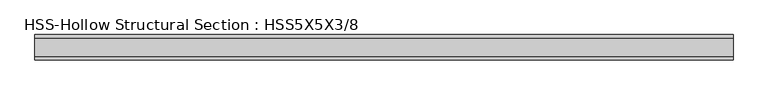
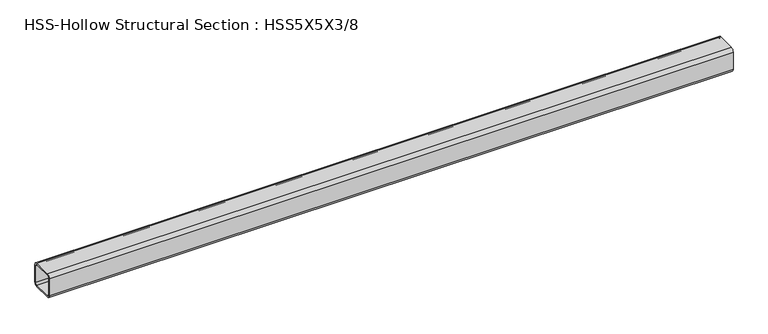
"""IFC4 building model written with IfcOpenShell, lengths in millimetres: member geometry, HSS-Hollow Structural Section : HSS5X5X3/8."""

import ifcopenshell
import ifcopenshell.guid

model = None  # the IFC model being written
_history = None  # IfcOwnerHistory: only IFC2X3 demands one
_inside = {}  # id of a spatial element -> (the spatial element, [elements in it])
_under = {}  # id of a project, library or spatial element -> (it, [spatial elements below it])
_declared = {}  # id of a project -> (the project, [libraries it declares])
_typed = {}  # id of a type object -> (the type object, [elements of that type])
_made_of = {}  # id of a material, layer set ... -> (it, [elements and type objects made of it])


def new_model(schema):
    """Start an empty IFC model of exactly this schema.

    Asked for "IFC4X3", IfcOpenShell would pick the latest addendum, in which some entities
    have other attributes; the version numbers below select the first issue.
    IFC2X3 requires an IfcOwnerHistory on every rooted entity: one is made here for all.
    """
    global model, _history
    if schema == "IFC4X3":
        model = ifcopenshell.file(schema_version=(4, 3, 0, 0))
    else:
        model = ifcopenshell.file(schema=schema)
    _inside.clear()
    _under.clear()
    _declared.clear()
    _typed.clear()
    _made_of.clear()
    _history = None
    if model.schema == "IFC2X3":
        org = make("IfcOrganization", Name="unknown")
        user = make(
            "IfcPersonAndOrganization",
            ThePerson=make("IfcPerson", FamilyName="unknown"),
            TheOrganization=org,
        )
        app = make(
            "IfcApplication",
            ApplicationDeveloper=org,
            Version="unknown",
            ApplicationFullName="unknown",
            ApplicationIdentifier="unknown",
        )
        _history = make(
            "IfcOwnerHistory",
            OwningUser=user,
            OwningApplication=app,
            ChangeAction="ADDED",
            CreationDate=0,
        )
    return model


def make(cls, **values):
    """One entity of the class cls with the attributes given. An attribute that is None is left unset."""
    return model.create_entity(
        cls, **{name: value for name, value in values.items() if value is not None}
    )


def rooted(cls, **values):
    """An entity with a GlobalId (a new one), such as an element, a storey or a relation."""
    return make(cls, GlobalId=ifcopenshell.guid.new(), OwnerHistory=_history, **values)


def si_unit(unit_type, name, prefix=None):
    """IfcSIUnit, for example si_unit("LENGTHUNIT", "METRE", prefix="MILLI")."""
    return make("IfcSIUnit", UnitType=unit_type, Prefix=prefix, Name=name)


def assignment(units):
    """IfcUnitAssignment: the units of a project."""
    return None if units is None else make("IfcUnitAssignment", Units=units)


def point(xyz):
    """IfcCartesianPoint."""
    return None if xyz is None else make("IfcCartesianPoint", Coordinates=xyz)


def direction(xyz):
    """IfcDirection."""
    return None if xyz is None else make("IfcDirection", DirectionRatios=xyz)


def frame(location, z_axis=None, x_axis=None):
    """IfcAxis2Placement3D, a coordinate frame: its origin and axes. An axis left out is left unset."""
    return make(
        "IfcAxis2Placement3D",
        Location=point(location),
        Axis=direction(z_axis),
        RefDirection=direction(x_axis),
    )


def frame_2d(location, x_axis=None):
    """IfcAxis2Placement2D, a coordinate frame in the plane: its origin and x axis."""
    return make(
        "IfcAxis2Placement2D", Location=point(location), RefDirection=direction(x_axis)
    )


def origin():
    """The frame at (0, 0, 0) with its axes left unset."""
    return frame((0.0, 0.0, 0.0))


def place(relative_to, where):
    """IfcLocalPlacement: puts the frame where relative to a parent placement (None: the world)."""
    return make(
        "IfcLocalPlacement", PlacementRelTo=relative_to, RelativePlacement=where
    )


def context(
    kind, dimensions, precision=None, world=None, true_north=None, identifier=None
):
    """IfcGeometricRepresentationContext, for example the 3D "Model" context."""
    return make(
        "IfcGeometricRepresentationContext",
        ContextIdentifier=identifier,
        ContextType=kind,
        CoordinateSpaceDimension=dimensions,
        Precision=precision,
        WorldCoordinateSystem=world,
        TrueNorth=true_north,
    )


def project(units=None, contexts=None):
    """IfcProject with its units and contexts."""
    return rooted(
        "IfcProject",
        Name="project",
        RepresentationContexts=contexts,
        UnitsInContext=assignment(units),
    )


def spatial(cls, under=None, at=None, **own):
    """A site, building, storey or space (cls), placed at a placement, below another one or the project."""
    s = rooted(cls, ObjectPlacement=at, **own)
    if under is not None:
        _under.setdefault(under.id(), (under, []))[1].append(s)
    return s


def polyline(points):
    """IfcPolyline through the points."""
    return make("IfcPolyline", Points=[point(p) for p in points])


def circle_curve(where, radius):
    """IfcCircle in the frame where."""
    return make("IfcCircle", Position=where, Radius=radius)


def trimmed(basis, trim1, trim2, sense, master):
    """IfcTrimmedCurve: the piece of a basis curve between two trims."""
    return make(
        "IfcTrimmedCurve",
        BasisCurve=basis,
        Trim1=trim1,
        Trim2=trim2,
        SenseAgreement=sense,
        MasterRepresentation=master,
    )


def segment(curve, same_sense, transition):
    """IfcCompositeCurveSegment."""
    return make(
        "IfcCompositeCurveSegment",
        Transition=transition,
        SameSense=same_sense,
        ParentCurve=curve,
    )


def composite_curve(segments, self_intersect=None):
    """IfcCompositeCurve: segments joined end to end."""
    return make("IfcCompositeCurve", Segments=segments, SelfIntersect=self_intersect)


def outline(outer, holes=None, kind="AREA"):
    """IfcArbitraryClosedProfileDef: a profile drawn as a closed curve; with holes, ...WithVoids."""
    if holes is None:
        return make("IfcArbitraryClosedProfileDef", ProfileType=kind, OuterCurve=outer)
    return make(
        "IfcArbitraryProfileDefWithVoids",
        ProfileType=kind,
        OuterCurve=outer,
        InnerCurves=holes,
    )


def extrude(swept, where, along, depth):
    """IfcExtrudedAreaSolid: the profile swept, set in the frame where, extruded along a direction by depth."""
    return make(
        "IfcExtrudedAreaSolid",
        SweptArea=swept,
        Position=where,
        ExtrudedDirection=direction(along),
        Depth=depth,
    )


def shape(context_of_items, identifier, shape_type, items):
    """IfcShapeRepresentation: the items that make up one representation, for example the "Body"."""
    return make(
        "IfcShapeRepresentation",
        ContextOfItems=context_of_items,
        RepresentationIdentifier=identifier,
        RepresentationType=shape_type,
        Items=items,
    )


def source(mapping_origin, context_of_items, identifier, shape_type, items):
    """IfcRepresentationMap: a shape defined once, which mapped items show again and again."""
    return make(
        "IfcRepresentationMap",
        MappingOrigin=mapping_origin,
        MappedRepresentation=shape(context_of_items, identifier, shape_type, items),
    )


def transform(
    local_origin,
    x_axis=None,
    y_axis=None,
    z_axis=None,
    scale=None,
    scale2=None,
    scale3=None,
    uniform=True,
):
    """IfcCartesianTransformationOperator3D, or its non-uniform kind. x_axis, y_axis, z_axis: its Axis1, 2, 3."""
    if uniform:
        return make(
            "IfcCartesianTransformationOperator3D",
            Axis1=direction(x_axis),
            Axis2=direction(y_axis),
            LocalOrigin=point(local_origin),
            Scale=scale,
            Axis3=direction(z_axis),
        )
    return make(
        "IfcCartesianTransformationOperator3DnonUniform",
        Axis1=direction(x_axis),
        Axis2=direction(y_axis),
        LocalOrigin=point(local_origin),
        Scale=scale,
        Axis3=direction(z_axis),
        Scale2=scale2,
        Scale3=scale3,
    )


def mapped(mapping_source, mapping_target):
    """IfcMappedItem: shows the shape of a source again, moved by a transform."""
    return make(
        "IfcMappedItem", MappingSource=mapping_source, MappingTarget=mapping_target
    )


def made_of(thing, what):
    """Note that an element or type object is made of a material, layer set ...; save() writes the relation."""
    if what is not None:
        _made_of.setdefault(what.id(), (what, []))[1].append(thing)
    return thing


def element(
    cls,
    number,
    at=None,
    inside=None,
    cuts=None,
    type_object=None,
    material=None,
    context=None,
    identifier="Body",
    shape_type=None,
    held_by="IfcProductDefinitionShape",
    body=None,
    shapes=None,
    **own,
):
    """One element of the class cls, such as IfcWall. Its Tag is "e" and its number.

    at: its placement. inside: the storey or other place that contains it. cuts: it is an
    opening in that element (IfcRelVoidsElement). A single representation is given by context,
    identifier, shape_type and body (its items); several are given by shapes. held_by: the class
    of the entity that holds the representations. save() writes the other relations.
    """
    e = rooted(cls, Tag="e%d" % number, ObjectPlacement=at, **own)
    if body is not None:
        shapes = [shape(context, identifier, shape_type, body)]
    if shapes is not None:
        e.Representation = make(held_by, Representations=shapes)
    if inside is not None:
        _inside.setdefault(inside.id(), (inside, []))[1].append(e)
    if cuts is not None:
        rooted(
            "IfcRelVoidsElement", RelatingBuildingElement=cuts, RelatedOpeningElement=e
        )
    if type_object is not None:
        _typed.setdefault(type_object.id(), (type_object, []))[1].append(e)
    return made_of(e, material)


def aggregate(whole, parts):
    """IfcRelAggregates: a whole, such as a stair, and the parts it consists of."""
    return rooted("IfcRelAggregates", RelatingObject=whole, RelatedObjects=parts)


def save(model, path):
    """Write the relations noted so far, then the file.

    IfcRelAggregates (storeys below a building ...), IfcRelContainedInSpatialStructure (elements
    in a storey), IfcRelDefinesByType, IfcRelAssociatesMaterial and IfcRelDeclares: one each for
    every whole, place, type object, material and project.
    """
    for whole, parts in _under.values():
        aggregate(whole, parts)
    for where, things in _inside.values():
        rooted(
            "IfcRelContainedInSpatialStructure",
            RelatedElements=things,
            RelatingStructure=where,
        )
    for kind, things in _typed.values():
        rooted("IfcRelDefinesByType", RelatedObjects=things, RelatingType=kind)
    for what, things in _made_of.values():
        rooted("IfcRelAssociatesMaterial", RelatedObjects=things, RelatingMaterial=what)
    for by, libraries in _declared.values():
        rooted("IfcRelDeclares", RelatingContext=by, RelatedDefinitions=libraries)
    model.write(path)


def hss_hollow_structural_section_hss5x5x3_8_885ac686(model_context):
    return source(origin(), model_context, "Body", "SweptSolid", [
        extrude(outline(composite_curve([segment(polyline([(63.5, 45.7708), (63.5, -45.7708)]), True, "CONTINUOUS"), segment(trimmed(circle_curve(frame_2d((45.7708, -45.7708)), 17.7292), [point((63.5, -45.7708))], [point((45.7708, -63.5))], False, "CARTESIAN"), True, "CONTINUOUS"), segment(polyline([(45.7708, -63.5), (-45.7708, -63.5)]), True, "CONTINUOUS"), segment(trimmed(circle_curve(frame_2d((-45.7708, -45.7708)), 17.7292), [point((-45.7708, -63.5))], [point((-63.5, -45.7708))], False, "CARTESIAN"), True, "CONTINUOUS"), segment(polyline([(-63.5, -45.7708), (-63.5, 45.7708)]), True, "CONTINUOUS"), segment(trimmed(circle_curve(frame_2d((-45.7708, 45.7708)), 17.7292), [point((-63.5, 45.7708))], [point((-45.7708, 63.5))], False, "CARTESIAN"), True, "CONTINUOUS"), segment(polyline([(-45.7708, 63.5), (45.7708, 63.5)]), True, "CONTINUOUS"), segment(trimmed(circle_curve(frame_2d((45.7708, 45.7708)), 17.7292), [point((45.7708, 63.5))], [point((63.5, 45.7708))], False, "CARTESIAN"), True, "CONTINUOUS")], self_intersect=False), holes=[composite_curve([segment(trimmed(circle_curve(frame_2d((-45.7708, 45.7708)), 8.8646), [point((-45.7708, 54.6354))], [point((-54.6354, 45.7708))], True, "CARTESIAN"), True, "CONTINUOUS"), segment(polyline([(-54.6354, 45.7708), (-54.6354, -45.7708)]), True, "CONTINUOUS"), segment(trimmed(circle_curve(frame_2d((-45.7708, -45.7708)), 8.8646), [point((-54.6354, -45.7708))], [point((-45.7708, -54.6354))], True, "CARTESIAN"), True, "CONTINUOUS"), segment(polyline([(-45.7708, -54.6354), (45.7708, -54.6354)]), True, "CONTINUOUS"), segment(trimmed(circle_curve(frame_2d((45.7708, -45.7708)), 8.8646), [point((45.7708, -54.6354))], [point((54.6354, -45.7708))], True, "CARTESIAN"), True, "CONTINUOUS"), segment(polyline([(54.6354, -45.7708), (54.6354, 45.7708)]), True, "CONTINUOUS"), segment(trimmed(circle_curve(frame_2d((45.7708, 45.7708)), 8.8646), [point((54.6354, 45.7708))], [point((45.7708, 54.6354))], True, "CARTESIAN"), True, "CONTINUOUS"), segment(polyline([(45.7708, 54.6354), (-45.7708, 54.6354)]), True, "CONTINUOUS")], self_intersect=False)]), frame((-1647.9284414, 0.0, 0.0), z_axis=(1.0, 0.0, 0.0), x_axis=(0.0, 1.0, 0.0)), (0.0, 0.0, 1.0), 3514.3211622),
    ])


if __name__ == "__main__":
    model = new_model("IFC4")
    model_context = context("Model", 3, world=origin())
    ifc_project = project(units=[si_unit("LENGTHUNIT", "METRE", prefix="MILLI")], contexts=[model_context])
    site = spatial("IfcSite", under=ifc_project)
    building = spatial("IfcBuilding", under=site)
    placement = place(None, origin())
    hss_hollow_structural_section_hss5x5x3_8_shape = hss_hollow_structural_section_hss5x5x3_8_885ac686(model_context)
    element("IfcMember", 1, ObjectType="HSS-Hollow Structural Section : HSS5X5X3/8", at=placement, inside=building, context=model_context, shape_type="MappedRepresentation", body=[
        mapped(hss_hollow_structural_section_hss5x5x3_8_shape, transform((0.0, 0.0, 0.0), x_axis=(1.0, 0.0, 0.0), y_axis=(0.0, 1.0, 0.0), z_axis=(0.0, 0.0, 1.0))),
    ])
    save(model, "model.ifc")

# Revit data of these elements
# Type "HSS-Hollow Structural Section : HSS5X5X3/8"
#   Assembly Code = "B10"
#   Shape = "Square"
#   W = 22.3
#   Ht = 0' - 5"
#   Length [instance default] = 5' - 0"
#   b = 0' - 5"
#   kr = 0' - 0.698"
#   t = 0' - 0.349"
#   A = 0.0429167 SF
#   Structural Material [instance default] = Steel ASTM A500, Grade B, Rectangular and Square
# Element 1 (IfcMember, "HSS-Hollow Structural Section : HSS5X5X3/8")
#   Materials on its faces: "Steel ASTM A500, Grade B, Rectangular and Square"
# Materials
#   "Steel ASTM A500, Grade B, Rectangular and Square": class "Metal", colour RGB 199 199 199, transparency 0, Description = "Carbon steel", Cost = 0
